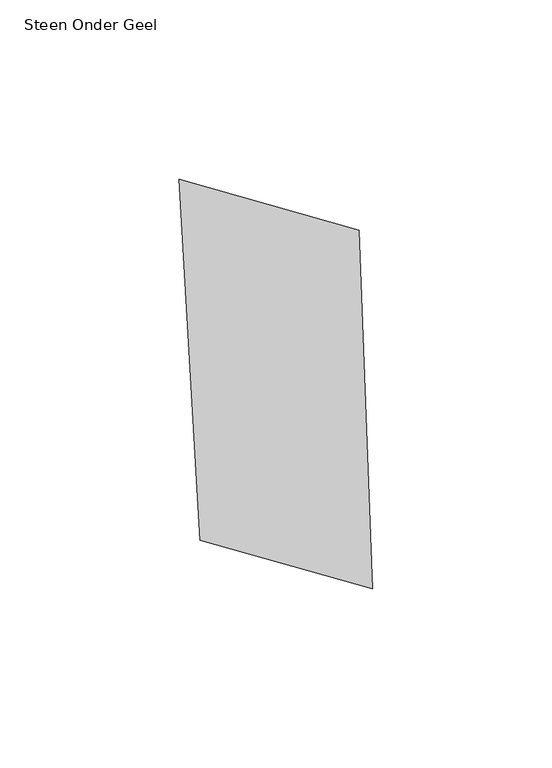
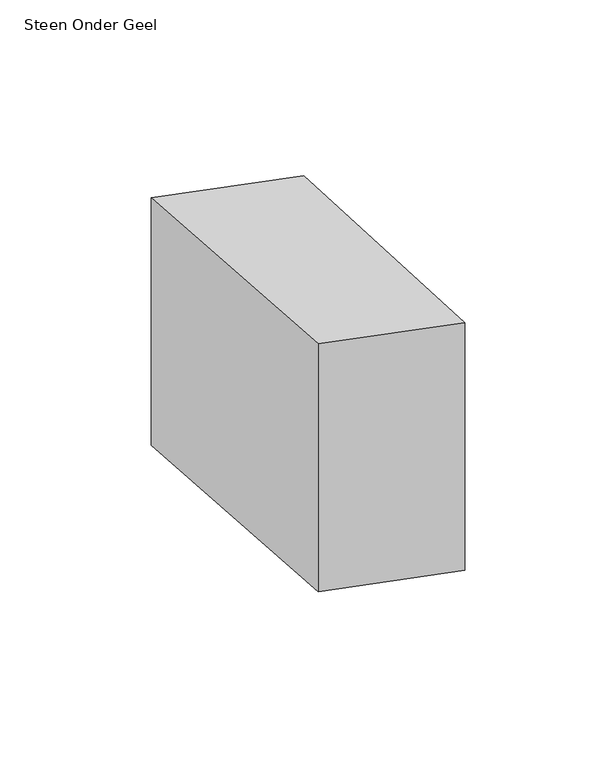
"""IFC4 building model written with IfcOpenShell, lengths in millimetres: proxy geometry, 00_GMA_steen_versie_4 : Steen Onder Geel."""

from ifc_helpers import new_model, si_unit, origin, origin_with_axes, place, context, project, spatial, polyline, outline, extrude, source, transform, mapped, element, save


def steen_onder_geel_3df0ab17(model_context):
    return source(origin(), model_context, "Body", "SweptSolid", [
        extrude(outline(polyline([(98.9532778, 117.4501682), (102.7150045, 17.4552989), (54.5816551, 30.9897246), (48.7791724, 131.585984), (98.9532778, 117.4501682)])), origin_with_axes(), (0.0, 0.0, 1.0), 100.0),
    ])


if __name__ == "__main__":
    model = new_model("IFC4")
    model_context = context("Model", 3, world=origin())
    ifc_project = project(units=[si_unit("LENGTHUNIT", "METRE", prefix="MILLI")], contexts=[model_context])
    site = spatial("IfcSite", under=ifc_project)
    building = spatial("IfcBuilding", under=site)
    placement = place(None, origin())
    steen_onder_geel_shape = steen_onder_geel_3df0ab17(model_context)
    element("IfcBuildingElementProxy", 1, Name="00_GMA_steen_versie_4 : Steen Onder Geel", ObjectType="00_GMA_steen_versie_4 : Steen Onder Geel", at=placement, inside=building, context=model_context, shape_type="MappedRepresentation", body=[
        mapped(steen_onder_geel_shape, transform((0.0, 0.0, 0.0), x_axis=(1.0, 0.0, 0.0), y_axis=(0.0, 1.0, 0.0), z_axis=(0.0, 0.0, 1.0))),
    ])
    save(model, "model.ifc")

# Revit data of these elements
# Type "00_GMA_steen_versie_4 : Steen Onder Geel"
#   StootVoegHalfBoven [instance default] = 5 mm
#   StootVoegHalf [instance default] = 5 mm
#   StootVoegBreedteOnder = 10 mm
#   StootVoegBreedteBoven = 10 mm
#   Steendikte = 100 mm
#   LintVoegOnderHalf = 0 mm
#   LintVoegOnder = 0 mm
#   LintVoegBovenHalf = 5 mm
#   LintVoegBoven = 10 mm
#   materiaal = 21_steen_geel
#   MateriaalVoeg = none
#   Default Elevation = 0
# Element 1 (IfcBuildingElementProxy, "00_GMA_steen_versie_4 : Steen Onder Geel")
#   Materials on its faces: "21_steen_geel"
# Materials
#   "21_steen_geel": class "Unassigned", colour RGB 202 202 0, transparency 0, Cost = 0
